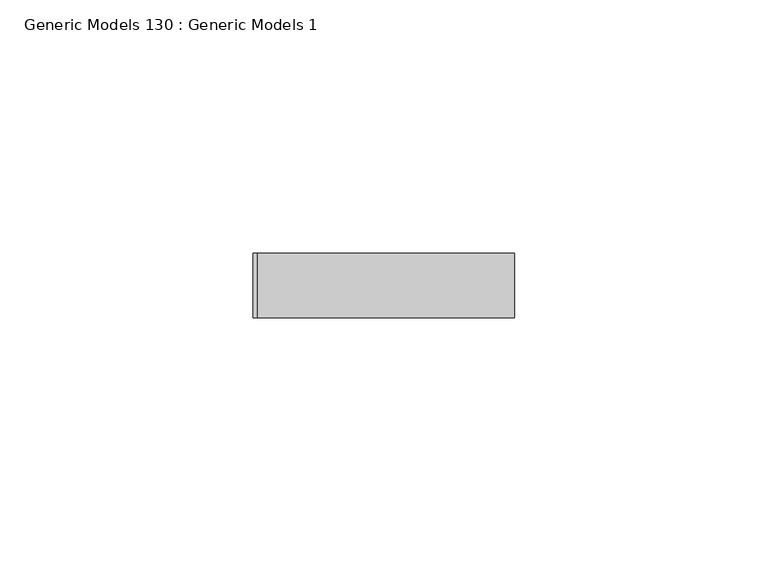
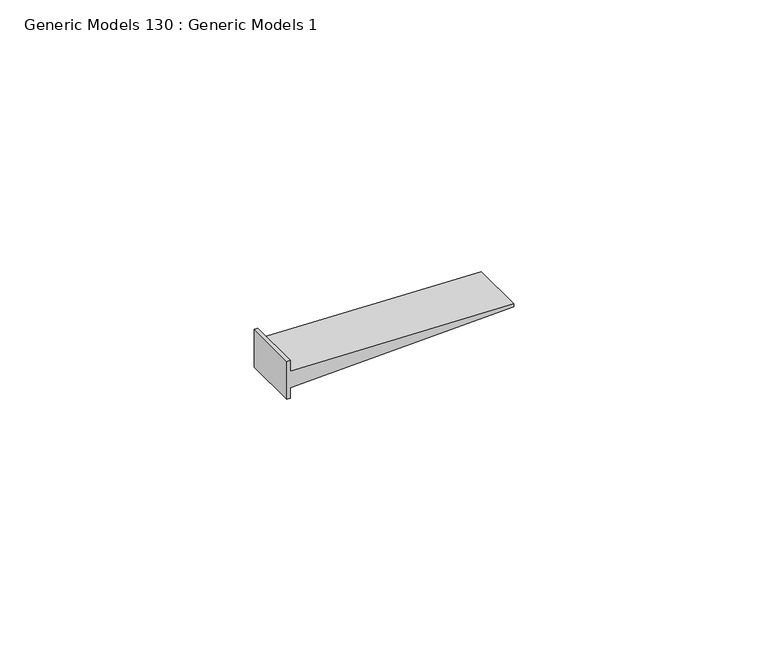
"""IFC4 building model written with IfcOpenShell, lengths in millimetres: proxy geometry, Generic Models 130 : Generic Models 1."""

import ifcopenshell
import ifcopenshell.guid

model = None  # the IFC model being written
_history = None  # IfcOwnerHistory: only IFC2X3 demands one
_inside = {}  # id of a spatial element -> (the spatial element, [elements in it])
_under = {}  # id of a project, library or spatial element -> (it, [spatial elements below it])
_declared = {}  # id of a project -> (the project, [libraries it declares])
_typed = {}  # id of a type object -> (the type object, [elements of that type])
_made_of = {}  # id of a material, layer set ... -> (it, [elements and type objects made of it])


def new_model(schema):
    """Start an empty IFC model of exactly this schema.

    Asked for "IFC4X3", IfcOpenShell would pick the latest addendum, in which some entities
    have other attributes; the version numbers below select the first issue.
    IFC2X3 requires an IfcOwnerHistory on every rooted entity: one is made here for all.
    """
    global model, _history
    if schema == "IFC4X3":
        model = ifcopenshell.file(schema_version=(4, 3, 0, 0))
    else:
        model = ifcopenshell.file(schema=schema)
    _inside.clear()
    _under.clear()
    _declared.clear()
    _typed.clear()
    _made_of.clear()
    _history = None
    if model.schema == "IFC2X3":
        org = make("IfcOrganization", Name="unknown")
        user = make(
            "IfcPersonAndOrganization",
            ThePerson=make("IfcPerson", FamilyName="unknown"),
            TheOrganization=org,
        )
        app = make(
            "IfcApplication",
            ApplicationDeveloper=org,
            Version="unknown",
            ApplicationFullName="unknown",
            ApplicationIdentifier="unknown",
        )
        _history = make(
            "IfcOwnerHistory",
            OwningUser=user,
            OwningApplication=app,
            ChangeAction="ADDED",
            CreationDate=0,
        )
    return model


def make(cls, **values):
    """One entity of the class cls with the attributes given. An attribute that is None is left unset."""
    return model.create_entity(
        cls, **{name: value for name, value in values.items() if value is not None}
    )


def rooted(cls, **values):
    """An entity with a GlobalId (a new one), such as an element, a storey or a relation."""
    return make(cls, GlobalId=ifcopenshell.guid.new(), OwnerHistory=_history, **values)


def si_unit(unit_type, name, prefix=None):
    """IfcSIUnit, for example si_unit("LENGTHUNIT", "METRE", prefix="MILLI")."""
    return make("IfcSIUnit", UnitType=unit_type, Prefix=prefix, Name=name)


def assignment(units):
    """IfcUnitAssignment: the units of a project."""
    return None if units is None else make("IfcUnitAssignment", Units=units)


def point(xyz):
    """IfcCartesianPoint."""
    return None if xyz is None else make("IfcCartesianPoint", Coordinates=xyz)


def direction(xyz):
    """IfcDirection."""
    return None if xyz is None else make("IfcDirection", DirectionRatios=xyz)


def frame(location, z_axis=None, x_axis=None):
    """IfcAxis2Placement3D, a coordinate frame: its origin and axes. An axis left out is left unset."""
    return make(
        "IfcAxis2Placement3D",
        Location=point(location),
        Axis=direction(z_axis),
        RefDirection=direction(x_axis),
    )


def origin():
    """The frame at (0, 0, 0) with its axes left unset."""
    return frame((0.0, 0.0, 0.0))


def place(relative_to, where):
    """IfcLocalPlacement: puts the frame where relative to a parent placement (None: the world)."""
    return make(
        "IfcLocalPlacement", PlacementRelTo=relative_to, RelativePlacement=where
    )


def context(
    kind, dimensions, precision=None, world=None, true_north=None, identifier=None
):
    """IfcGeometricRepresentationContext, for example the 3D "Model" context."""
    return make(
        "IfcGeometricRepresentationContext",
        ContextIdentifier=identifier,
        ContextType=kind,
        CoordinateSpaceDimension=dimensions,
        Precision=precision,
        WorldCoordinateSystem=world,
        TrueNorth=true_north,
    )


def project(units=None, contexts=None):
    """IfcProject with its units and contexts."""
    return rooted(
        "IfcProject",
        Name="project",
        RepresentationContexts=contexts,
        UnitsInContext=assignment(units),
    )


def spatial(cls, under=None, at=None, **own):
    """A site, building, storey or space (cls), placed at a placement, below another one or the project."""
    s = rooted(cls, ObjectPlacement=at, **own)
    if under is not None:
        _under.setdefault(under.id(), (under, []))[1].append(s)
    return s


def polyline(points):
    """IfcPolyline through the points."""
    return make("IfcPolyline", Points=[point(p) for p in points])


def outline(outer, holes=None, kind="AREA"):
    """IfcArbitraryClosedProfileDef: a profile drawn as a closed curve; with holes, ...WithVoids."""
    if holes is None:
        return make("IfcArbitraryClosedProfileDef", ProfileType=kind, OuterCurve=outer)
    return make(
        "IfcArbitraryProfileDefWithVoids",
        ProfileType=kind,
        OuterCurve=outer,
        InnerCurves=holes,
    )


def extrude(swept, where, along, depth):
    """IfcExtrudedAreaSolid: the profile swept, set in the frame where, extruded along a direction by depth."""
    return make(
        "IfcExtrudedAreaSolid",
        SweptArea=swept,
        Position=where,
        ExtrudedDirection=direction(along),
        Depth=depth,
    )


def shape(context_of_items, identifier, shape_type, items):
    """IfcShapeRepresentation: the items that make up one representation, for example the "Body"."""
    return make(
        "IfcShapeRepresentation",
        ContextOfItems=context_of_items,
        RepresentationIdentifier=identifier,
        RepresentationType=shape_type,
        Items=items,
    )


def source(mapping_origin, context_of_items, identifier, shape_type, items):
    """IfcRepresentationMap: a shape defined once, which mapped items show again and again."""
    return make(
        "IfcRepresentationMap",
        MappingOrigin=mapping_origin,
        MappedRepresentation=shape(context_of_items, identifier, shape_type, items),
    )


def transform(
    local_origin,
    x_axis=None,
    y_axis=None,
    z_axis=None,
    scale=None,
    scale2=None,
    scale3=None,
    uniform=True,
):
    """IfcCartesianTransformationOperator3D, or its non-uniform kind. x_axis, y_axis, z_axis: its Axis1, 2, 3."""
    if uniform:
        return make(
            "IfcCartesianTransformationOperator3D",
            Axis1=direction(x_axis),
            Axis2=direction(y_axis),
            LocalOrigin=point(local_origin),
            Scale=scale,
            Axis3=direction(z_axis),
        )
    return make(
        "IfcCartesianTransformationOperator3DnonUniform",
        Axis1=direction(x_axis),
        Axis2=direction(y_axis),
        LocalOrigin=point(local_origin),
        Scale=scale,
        Axis3=direction(z_axis),
        Scale2=scale2,
        Scale3=scale3,
    )


def mapped(mapping_source, mapping_target):
    """IfcMappedItem: shows the shape of a source again, moved by a transform."""
    return make(
        "IfcMappedItem", MappingSource=mapping_source, MappingTarget=mapping_target
    )


def made_of(thing, what):
    """Note that an element or type object is made of a material, layer set ...; save() writes the relation."""
    if what is not None:
        _made_of.setdefault(what.id(), (what, []))[1].append(thing)
    return thing


def element(
    cls,
    number,
    at=None,
    inside=None,
    cuts=None,
    type_object=None,
    material=None,
    context=None,
    identifier="Body",
    shape_type=None,
    held_by="IfcProductDefinitionShape",
    body=None,
    shapes=None,
    **own,
):
    """One element of the class cls, such as IfcWall. Its Tag is "e" and its number.

    at: its placement. inside: the storey or other place that contains it. cuts: it is an
    opening in that element (IfcRelVoidsElement). A single representation is given by context,
    identifier, shape_type and body (its items); several are given by shapes. held_by: the class
    of the entity that holds the representations. save() writes the other relations.
    """
    e = rooted(cls, Tag="e%d" % number, ObjectPlacement=at, **own)
    if body is not None:
        shapes = [shape(context, identifier, shape_type, body)]
    if shapes is not None:
        e.Representation = make(held_by, Representations=shapes)
    if inside is not None:
        _inside.setdefault(inside.id(), (inside, []))[1].append(e)
    if cuts is not None:
        rooted(
            "IfcRelVoidsElement", RelatingBuildingElement=cuts, RelatedOpeningElement=e
        )
    if type_object is not None:
        _typed.setdefault(type_object.id(), (type_object, []))[1].append(e)
    return made_of(e, material)


def aggregate(whole, parts):
    """IfcRelAggregates: a whole, such as a stair, and the parts it consists of."""
    return rooted("IfcRelAggregates", RelatingObject=whole, RelatedObjects=parts)


def save(model, path):
    """Write the relations noted so far, then the file.

    IfcRelAggregates (storeys below a building ...), IfcRelContainedInSpatialStructure (elements
    in a storey), IfcRelDefinesByType, IfcRelAssociatesMaterial and IfcRelDeclares: one each for
    every whole, place, type object, material and project.
    """
    for whole, parts in _under.values():
        aggregate(whole, parts)
    for where, things in _inside.values():
        rooted(
            "IfcRelContainedInSpatialStructure",
            RelatedElements=things,
            RelatingStructure=where,
        )
    for kind, things in _typed.values():
        rooted("IfcRelDefinesByType", RelatedObjects=things, RelatingType=kind)
    for what, things in _made_of.values():
        rooted("IfcRelAssociatesMaterial", RelatedObjects=things, RelatingMaterial=what)
    for by, libraries in _declared.values():
        rooted("IfcRelDeclares", RelatingContext=by, RelatedDefinitions=libraries)
    model.write(path)


def generic_models_130_generic_models_1_e19555d7(model_context):
    return source(origin(), model_context, "Body", "SweptSolid", [
        extrude(outline(polyline([(2183.633033, 46827.1298031), (2174.539833, 46827.1298031), (2174.539833, 46827.9235531), (2177.0896966, 46827.9235531), (2178.6870857, 46878.7235531), (2179.4857803, 46878.7235531), (2181.0831694, 46827.9235531), (2183.633033, 46827.9235531), (2183.633033, 46827.1298031)])), frame((0.0, 565.15, 0.0), z_axis=(0.0, 1.0, 0.0), x_axis=(0.0, 0.0, 1.0)), (0.0, 0.0, 1.0), 12.7),
    ])


if __name__ == "__main__":
    model = new_model("IFC4")
    model_context = context("Model", 3, world=origin())
    ifc_project = project(units=[si_unit("LENGTHUNIT", "METRE", prefix="MILLI")], contexts=[model_context])
    site = spatial("IfcSite", under=ifc_project)
    building = spatial("IfcBuilding", under=site)
    placement = place(None, origin())
    generic_models_130_generic_models_1_shape = generic_models_130_generic_models_1_e19555d7(model_context)
    element("IfcBuildingElementProxy", 1, Name="Generic Models 130 : Generic Models 1", ObjectType="Generic Models 130 : Generic Models 1", at=placement, inside=building, context=model_context, shape_type="MappedRepresentation", body=[
        mapped(generic_models_130_generic_models_1_shape, transform((0.0, 0.0, 0.0), x_axis=(1.0, 0.0, 0.0), y_axis=(0.0, 1.0, 0.0), z_axis=(0.0, 0.0, 1.0))),
    ])
    save(model, "model.ifc")

# Revit data of these elements
# Element 1 (IfcBuildingElementProxy, "Generic Models 130 : Generic Models 1")
#   Materials on its faces: "ATTACH GYPSUM BOARD TO STUDS AND NOT TO TOP TRACK"
# Materials
#   "ATTACH GYPSUM BOARD TO STUDS AND NOT TO TOP TRACK": class "Generic", colour RGB 48 48 48, transparency 0, Cost = 0
